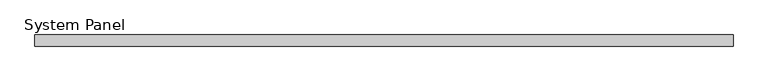
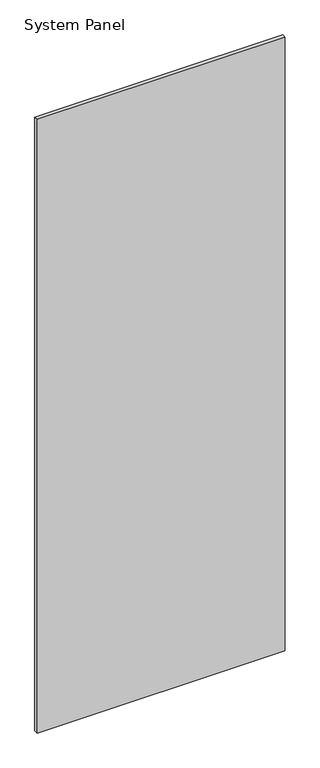
"""IFC4 building model written with IfcOpenShell, lengths in millimetres: plate geometry, System Panel : WWm-Glass-20mm-10mmOffset."""

from ifc_helpers import new_model, si_unit, origin, origin_with_axes, place, context, project, spatial, polyline, outline, extrude, source, transform, mapped, element, save


def system_panel_e7a82d1a(model_context):
    return source(origin(), model_context, "Body", "SweptSolid", [
        extrude(outline(polyline([(602.5, 0.0), (-602.5, 0.0), (-602.5, 20.0), (602.5, 20.0), (602.5, 0.0)])), origin_with_axes(), (0.0, 0.0, 1.0), 3150.0),
    ])


if __name__ == "__main__":
    model = new_model("IFC4")
    model_context = context("Model", 3, world=origin())
    ifc_project = project(units=[si_unit("LENGTHUNIT", "METRE", prefix="MILLI")], contexts=[model_context])
    site = spatial("IfcSite", under=ifc_project)
    building = spatial("IfcBuilding", under=site)
    placement = place(None, origin())
    system_panel_shape = system_panel_e7a82d1a(model_context)
    element("IfcPlate", 1, ObjectType="System Panel : WWm-Glass-20mm-10mmOffset", at=placement, inside=building, context=model_context, shape_type="MappedRepresentation", body=[
        mapped(system_panel_shape, transform((0.0, 0.0, 0.0), x_axis=(1.0, 0.0, 0.0), y_axis=(0.0, 1.0, 0.0), z_axis=(0.0, 0.0, 1.0))),
    ])
    save(model, "model.ifc")

# Revit data of these elements
# Type "System Panel : WWm-Glass-20mm-10mmOffset"
#   Finish = ""
# Element 1 (IfcPlate, "System Panel : WWm-Glass-20mm-10mmOffset")
#   Materials on its faces: "WW-EC-GL-Storefront"
# Materials
#   "WW-EC-GL-Storefront": class "Glass", colour RGB 236 240 239, transparency 0.85, Description = "Storefront Glass", Cost = 0
